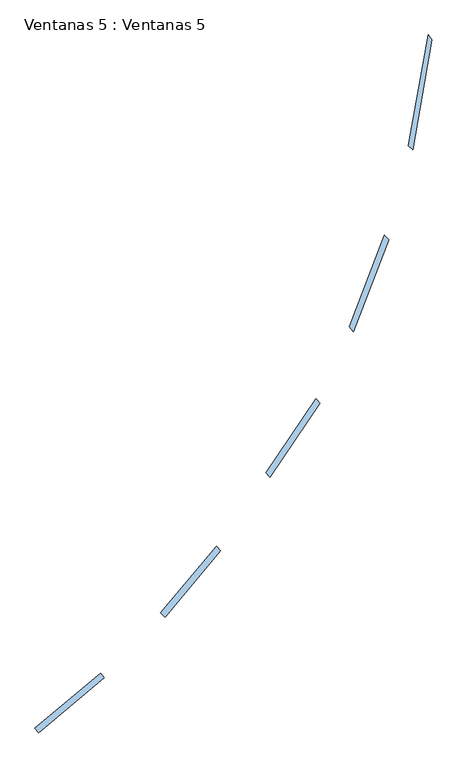
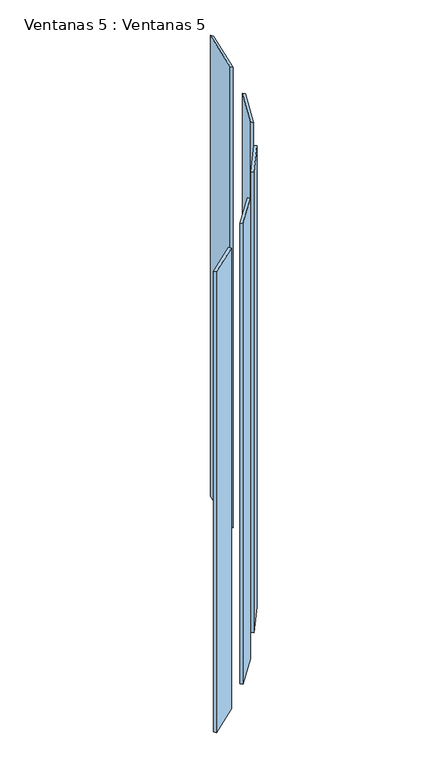
"""IFC4 building model written with IfcOpenShell, lengths in millimetres: window geometry, Ventanas 5 : Ventanas 5."""

from ifc_helpers import new_model, si_unit, frame, origin, place, context, project, spatial, polyline, outline, extrude, source, transform, mapped, element, save


def ventanas_5_ventanas_5_e1f55a8b(model_context):
    return source(origin(), model_context, "Body", "SweptSolid", [
        extrude(outline(polyline([(-3177.2970262, 5280.5240764), (-3164.441274, 5265.2031875), (-3378.9337181, 5085.2226568), (-3391.7894703, 5100.5435457), (-3177.2970262, 5280.5240764)])), frame((0.0, 0.0, 6206.6549752), z_axis=(0.0, 0.0, 1.0), x_axis=(1.0, 0.0, 0.0)), (0.0, 0.0, 1.0), 3564.0972111),
        extrude(outline(polyline([(-2797.3063962, 5695.5590216), (-2784.301998, 5680.0609834), (-2965.9212811, 5463.6155503), (-2980.0634167, 5477.7576859), (-2797.3063962, 5695.5590216)])), frame((0.0, 0.0, 6206.6549752), z_axis=(0.0, 0.0, 1.0), x_axis=(1.0, 0.0, 0.0)), (0.0, 0.0, 1.0), 3564.0972111),
        extrude(outline(polyline([(-2472.3466056, 6177.3317235), (-2459.4908534, 6162.0108346), (-2622.3747108, 5920.5255853), (-2635.230463, 5935.8464742), (-2472.3466056, 6177.3317235)])), frame((0.0, 0.0, 6206.6549752), z_axis=(0.0, 0.0, 1.0), x_axis=(1.0, 0.0, 0.0)), (0.0, 0.0, 1.0), 3564.0972111),
        extrude(outline(polyline([(-2248.3355774, 6710.566411), (-2234.1934418, 6696.4242754), (-2349.635275, 6395.688018), (-2363.0631842, 6411.690777), (-2248.3355774, 6710.566411)])), frame((0.0, 0.0, 6206.6549752), z_axis=(0.0, 0.0, 1.0), x_axis=(1.0, 0.0, 0.0)), (0.0, 0.0, 1.0), 3564.0972111),
        extrude(outline(polyline([(-2105.7958961, 7365.6163787), (-2092.9401439, 7350.2954898), (-2156.4109911, 6990.3344284), (-2169.636258, 7003.5596953), (-2105.7958961, 7365.6163787)])), frame((0.0, 0.0, 6206.6549752), z_axis=(0.0, 0.0, 1.0), x_axis=(1.0, 0.0, 0.0)), (0.0, 0.0, 1.0), 3564.0972111),
    ])


if __name__ == "__main__":
    model = new_model("IFC4")
    model_context = context("Model", 3, world=origin())
    ifc_project = project(units=[si_unit("LENGTHUNIT", "METRE", prefix="MILLI")], contexts=[model_context])
    site = spatial("IfcSite", under=ifc_project)
    building = spatial("IfcBuilding", under=site)
    placement = place(None, origin())
    ventanas_5_ventanas_5_shape = ventanas_5_ventanas_5_e1f55a8b(model_context)
    element("IfcWindow", 1, ObjectType="Ventanas 5 : Ventanas 5", at=placement, inside=building, context=model_context, shape_type="MappedRepresentation", body=[
        mapped(ventanas_5_ventanas_5_shape, transform((0.0, 0.0, 0.0), x_axis=(1.0, 0.0, 0.0), y_axis=(0.0, 1.0, 0.0), z_axis=(0.0, 0.0, 1.0))),
    ])
    save(model, "model.ifc")

# Revit data of these elements
# Type "Ventanas 5 : Ventanas 5"
#   Type Mark = "31"
# Element 1 (IfcWindow, "Ventanas 5 : Ventanas 5")
#   Materials on its faces: "VIDRIO"
# Materials
#   "VIDRIO": class "Genérico", colour RGB 120 120 120, transparency 0, Cost = 0
